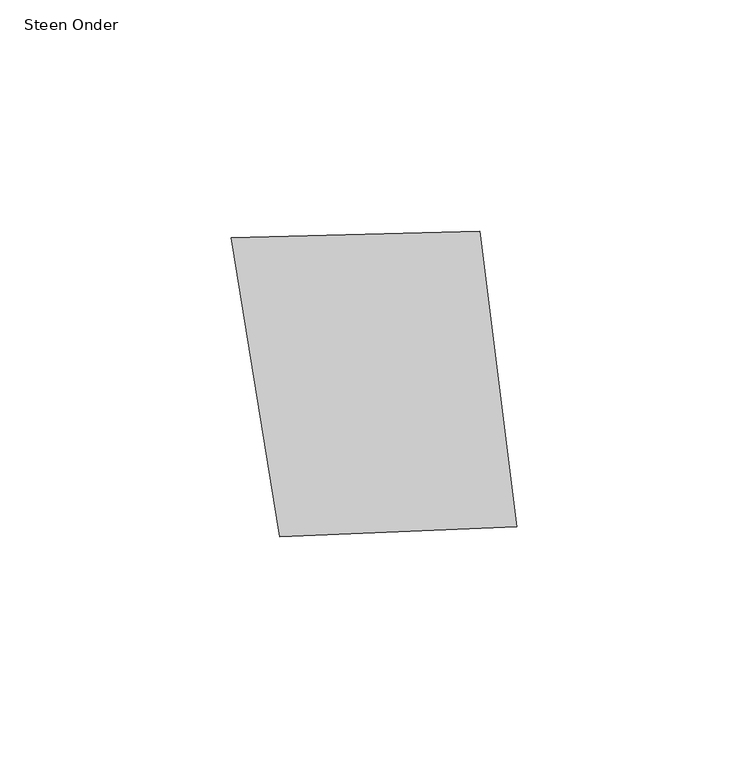
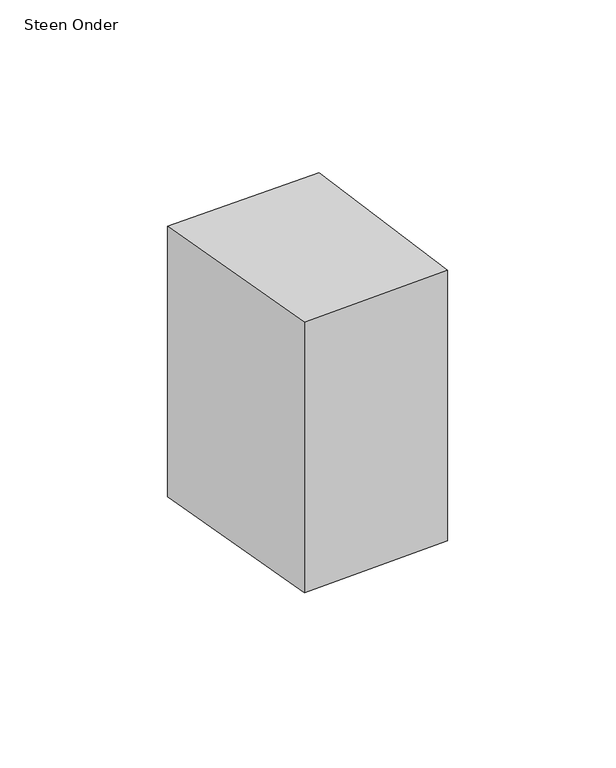
"""IFC4 building model written with IfcOpenShell, lengths in millimetres: proxy geometry, 00_GMA_steen_versie_4 : Steen Onder."""

from ifc_helpers import new_model, si_unit, origin, origin_with_axes, place, context, project, spatial, polyline, outline, extrude, source, transform, mapped, element, save


def steen_onder_9f632a0d(model_context):
    return source(origin(), model_context, "Body", "SweptSolid", [
        extrude(outline(polyline([(96.8538067, 98.0246627), (104.8765147, 33.9641043), (53.6279486, 31.8144658), (43.0565895, 96.5837311), (96.8538067, 98.0246627)])), origin_with_axes(), (0.0, 0.0, 1.0), 100.0),
    ])


if __name__ == "__main__":
    model = new_model("IFC4")
    model_context = context("Model", 3, world=origin())
    ifc_project = project(units=[si_unit("LENGTHUNIT", "METRE", prefix="MILLI")], contexts=[model_context])
    site = spatial("IfcSite", under=ifc_project)
    building = spatial("IfcBuilding", under=site)
    placement = place(None, origin())
    steen_onder_shape = steen_onder_9f632a0d(model_context)
    element("IfcBuildingElementProxy", 1, Name="00_GMA_steen_versie_4 : Steen Onder", ObjectType="00_GMA_steen_versie_4 : Steen Onder", at=placement, inside=building, context=model_context, shape_type="MappedRepresentation", body=[
        mapped(steen_onder_shape, transform((0.0, 0.0, 0.0), x_axis=(1.0, 0.0, 0.0), y_axis=(0.0, 1.0, 0.0), z_axis=(0.0, 0.0, 1.0))),
    ])
    save(model, "model.ifc")

# Revit data of these elements
# Type "00_GMA_steen_versie_4 : Steen Onder"
#   StootVoegHalfBoven [instance default] = 5 mm
#   StootVoegHalf [instance default] = 5 mm
#   StootVoegBreedteOnder = 10 mm
#   StootVoegBreedteBoven = 10 mm
#   Steendikte = 100 mm
#   LintVoegOnderHalf = 0 mm
#   LintVoegOnder = 0 mm
#   LintVoegBovenHalf = 5 mm
#   LintVoegBoven = 10 mm
#   materiaal = none
#   MateriaalVoeg = none
#   Default Elevation = 0
